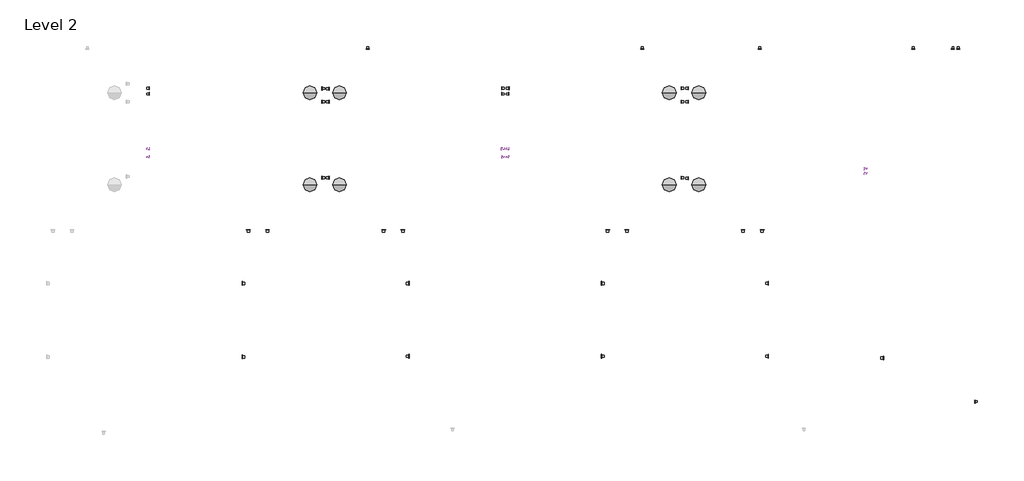
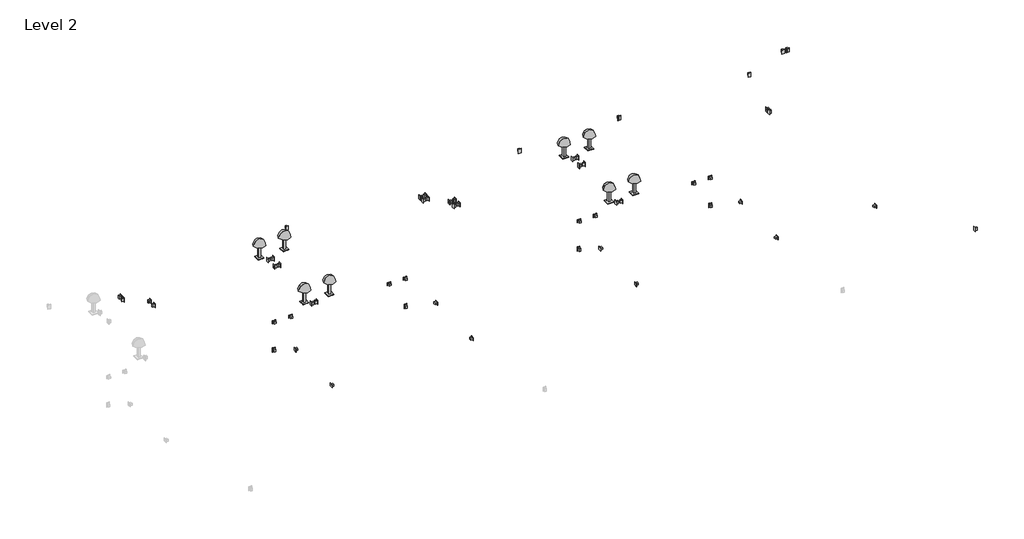
# One storey, part 2 of 2: 37 proxies, 17 switching devices, 8 light fixtures.
"""IFC4 building model written with IfcOpenShell, lengths in millimetres."""

import ifcopenshell
import ifcopenshell.guid

model = None  # the IFC model being written
_history = None  # IfcOwnerHistory: only IFC2X3 demands one
_inside = {}  # id of a spatial element -> (the spatial element, [elements in it])
_under = {}  # id of a project, library or spatial element -> (it, [spatial elements below it])
_declared = {}  # id of a project -> (the project, [libraries it declares])
_typed = {}  # id of a type object -> (the type object, [elements of that type])
_made_of = {}  # id of a material, layer set ... -> (it, [elements and type objects made of it])


def new_model(schema):
    """Start an empty IFC model of exactly this schema.

    Asked for "IFC4X3", IfcOpenShell would pick the latest addendum, in which some entities
    have other attributes; the version numbers below select the first issue.
    IFC2X3 requires an IfcOwnerHistory on every rooted entity: one is made here for all.
    """
    global model, _history
    if schema == "IFC4X3":
        model = ifcopenshell.file(schema_version=(4, 3, 0, 0))
    else:
        model = ifcopenshell.file(schema=schema)
    _inside.clear()
    _under.clear()
    _declared.clear()
    _typed.clear()
    _made_of.clear()
    _history = None
    if model.schema == "IFC2X3":
        org = make("IfcOrganization", Name="unknown")
        user = make(
            "IfcPersonAndOrganization",
            ThePerson=make("IfcPerson", FamilyName="unknown"),
            TheOrganization=org,
        )
        app = make(
            "IfcApplication",
            ApplicationDeveloper=org,
            Version="unknown",
            ApplicationFullName="unknown",
            ApplicationIdentifier="unknown",
        )
        _history = make(
            "IfcOwnerHistory",
            OwningUser=user,
            OwningApplication=app,
            ChangeAction="ADDED",
            CreationDate=0,
        )
    return model


def make(cls, **values):
    """One entity of the class cls with the attributes given. An attribute that is None is left unset."""
    return model.create_entity(
        cls, **{name: value for name, value in values.items() if value is not None}
    )


def rooted(cls, **values):
    """An entity with a GlobalId (a new one), such as an element, a storey or a relation."""
    return make(cls, GlobalId=ifcopenshell.guid.new(), OwnerHistory=_history, **values)


def si_unit(unit_type, name, prefix=None):
    """IfcSIUnit, for example si_unit("LENGTHUNIT", "METRE", prefix="MILLI")."""
    return make("IfcSIUnit", UnitType=unit_type, Prefix=prefix, Name=name)


def assignment(units):
    """IfcUnitAssignment: the units of a project."""
    return None if units is None else make("IfcUnitAssignment", Units=units)


def point(xyz):
    """IfcCartesianPoint."""
    return None if xyz is None else make("IfcCartesianPoint", Coordinates=xyz)


def direction(xyz):
    """IfcDirection."""
    return None if xyz is None else make("IfcDirection", DirectionRatios=xyz)


def frame(location, z_axis=None, x_axis=None):
    """IfcAxis2Placement3D, a coordinate frame: its origin and axes. An axis left out is left unset."""
    return make(
        "IfcAxis2Placement3D",
        Location=point(location),
        Axis=direction(z_axis),
        RefDirection=direction(x_axis),
    )


def frame_2d(location, x_axis=None):
    """IfcAxis2Placement2D, a coordinate frame in the plane: its origin and x axis."""
    return make(
        "IfcAxis2Placement2D", Location=point(location), RefDirection=direction(x_axis)
    )


def origin():
    """The frame at (0, 0, 0) with its axes left unset."""
    return frame((0.0, 0.0, 0.0))


def origin_with_axes():
    """The frame at (0, 0, 0) with the z axis (0, 0, 1) and the x axis (1, 0, 0) written out."""
    return frame((0.0, 0.0, 0.0), z_axis=(0.0, 0.0, 1.0), x_axis=(1.0, 0.0, 0.0))


def origin_2d():
    """The frame at (0, 0) in the plane with its x axis left unset."""
    return frame_2d((0.0, 0.0))


def place(relative_to, where):
    """IfcLocalPlacement: puts the frame where relative to a parent placement (None: the world)."""
    return make(
        "IfcLocalPlacement", PlacementRelTo=relative_to, RelativePlacement=where
    )


def context(
    kind, dimensions, precision=None, world=None, true_north=None, identifier=None
):
    """IfcGeometricRepresentationContext, for example the 3D "Model" context."""
    return make(
        "IfcGeometricRepresentationContext",
        ContextIdentifier=identifier,
        ContextType=kind,
        CoordinateSpaceDimension=dimensions,
        Precision=precision,
        WorldCoordinateSystem=world,
        TrueNorth=true_north,
    )


def project(units=None, contexts=None):
    """IfcProject with its units and contexts."""
    return rooted(
        "IfcProject",
        Name="project",
        RepresentationContexts=contexts,
        UnitsInContext=assignment(units),
    )


def spatial(cls, under=None, at=None, **own):
    """A site, building, storey or space (cls), placed at a placement, below another one or the project."""
    s = rooted(cls, ObjectPlacement=at, **own)
    if under is not None:
        _under.setdefault(under.id(), (under, []))[1].append(s)
    return s


def polyline(points):
    """IfcPolyline through the points."""
    return make("IfcPolyline", Points=[point(p) for p in points])


def circle_curve(where, radius):
    """IfcCircle in the frame where."""
    return make("IfcCircle", Position=where, Radius=radius)


def ellipse_curve(where, semi_axis1, semi_axis2):
    """IfcEllipse in the frame where."""
    return make(
        "IfcEllipse", Position=where, SemiAxis1=semi_axis1, SemiAxis2=semi_axis2
    )


def trimmed(basis, trim1, trim2, sense, master):
    """IfcTrimmedCurve: the piece of a basis curve between two trims."""
    return make(
        "IfcTrimmedCurve",
        BasisCurve=basis,
        Trim1=trim1,
        Trim2=trim2,
        SenseAgreement=sense,
        MasterRepresentation=master,
    )


def segment(curve, same_sense, transition):
    """IfcCompositeCurveSegment."""
    return make(
        "IfcCompositeCurveSegment",
        Transition=transition,
        SameSense=same_sense,
        ParentCurve=curve,
    )


def composite_curve(segments, self_intersect=None):
    """IfcCompositeCurve: segments joined end to end."""
    return make("IfcCompositeCurve", Segments=segments, SelfIntersect=self_intersect)


def outline(outer, holes=None, kind="AREA"):
    """IfcArbitraryClosedProfileDef: a profile drawn as a closed curve; with holes, ...WithVoids."""
    if holes is None:
        return make("IfcArbitraryClosedProfileDef", ProfileType=kind, OuterCurve=outer)
    return make(
        "IfcArbitraryProfileDefWithVoids",
        ProfileType=kind,
        OuterCurve=outer,
        InnerCurves=holes,
    )


def extrude(swept, where, along, depth):
    """IfcExtrudedAreaSolid: the profile swept, set in the frame where, extruded along a direction by depth."""
    return make(
        "IfcExtrudedAreaSolid",
        SweptArea=swept,
        Position=where,
        ExtrudedDirection=direction(along),
        Depth=depth,
    )


def shape(context_of_items, identifier, shape_type, items):
    """IfcShapeRepresentation: the items that make up one representation, for example the "Body"."""
    return make(
        "IfcShapeRepresentation",
        ContextOfItems=context_of_items,
        RepresentationIdentifier=identifier,
        RepresentationType=shape_type,
        Items=items,
    )


def source(mapping_origin, context_of_items, identifier, shape_type, items):
    """IfcRepresentationMap: a shape defined once, which mapped items show again and again."""
    return make(
        "IfcRepresentationMap",
        MappingOrigin=mapping_origin,
        MappedRepresentation=shape(context_of_items, identifier, shape_type, items),
    )


def transform(
    local_origin,
    x_axis=None,
    y_axis=None,
    z_axis=None,
    scale=None,
    scale2=None,
    scale3=None,
    uniform=True,
):
    """IfcCartesianTransformationOperator3D, or its non-uniform kind. x_axis, y_axis, z_axis: its Axis1, 2, 3."""
    if uniform:
        return make(
            "IfcCartesianTransformationOperator3D",
            Axis1=direction(x_axis),
            Axis2=direction(y_axis),
            LocalOrigin=point(local_origin),
            Scale=scale,
            Axis3=direction(z_axis),
        )
    return make(
        "IfcCartesianTransformationOperator3DnonUniform",
        Axis1=direction(x_axis),
        Axis2=direction(y_axis),
        LocalOrigin=point(local_origin),
        Scale=scale,
        Axis3=direction(z_axis),
        Scale2=scale2,
        Scale3=scale3,
    )


def mapped(mapping_source, mapping_target):
    """IfcMappedItem: shows the shape of a source again, moved by a transform."""
    return make(
        "IfcMappedItem", MappingSource=mapping_source, MappingTarget=mapping_target
    )


def made_of(thing, what):
    """Note that an element or type object is made of a material, layer set ...; save() writes the relation."""
    if what is not None:
        _made_of.setdefault(what.id(), (what, []))[1].append(thing)
    return thing


def element(
    cls,
    number,
    at=None,
    inside=None,
    cuts=None,
    type_object=None,
    material=None,
    context=None,
    identifier="Body",
    shape_type=None,
    held_by="IfcProductDefinitionShape",
    body=None,
    shapes=None,
    **own,
):
    """One element of the class cls, such as IfcWall. Its Tag is "e" and its number.

    at: its placement. inside: the storey or other place that contains it. cuts: it is an
    opening in that element (IfcRelVoidsElement). A single representation is given by context,
    identifier, shape_type and body (its items); several are given by shapes. held_by: the class
    of the entity that holds the representations. save() writes the other relations.
    """
    e = rooted(cls, Tag="e%d" % number, ObjectPlacement=at, **own)
    if body is not None:
        shapes = [shape(context, identifier, shape_type, body)]
    if shapes is not None:
        e.Representation = make(held_by, Representations=shapes)
    if inside is not None:
        _inside.setdefault(inside.id(), (inside, []))[1].append(e)
    if cuts is not None:
        rooted(
            "IfcRelVoidsElement", RelatingBuildingElement=cuts, RelatedOpeningElement=e
        )
    if type_object is not None:
        _typed.setdefault(type_object.id(), (type_object, []))[1].append(e)
    return made_of(e, material)


def aggregate(whole, parts):
    """IfcRelAggregates: a whole, such as a stair, and the parts it consists of."""
    return rooted("IfcRelAggregates", RelatingObject=whole, RelatedObjects=parts)


def save(model, path):
    """Write the relations noted so far, then the file.

    IfcRelAggregates (storeys below a building ...), IfcRelContainedInSpatialStructure (elements
    in a storey), IfcRelDefinesByType, IfcRelAssociatesMaterial and IfcRelDeclares: one each for
    every whole, place, type object, material and project.
    """
    for whole, parts in _under.values():
        aggregate(whole, parts)
    for where, things in _inside.values():
        rooted(
            "IfcRelContainedInSpatialStructure",
            RelatedElements=things,
            RelatingStructure=where,
        )
    for kind, things in _typed.values():
        rooted("IfcRelDefinesByType", RelatedObjects=things, RelatingType=kind)
    for what, things in _made_of.values():
        rooted("IfcRelAssociatesMaterial", RelatedObjects=things, RelatingMaterial=what)
    for by, libraries in _declared.values():
        rooted("IfcRelDeclares", RelatingContext=by, RelatedDefinitions=libraries)
    model.write(path)


def plane_surface(at):
    """IfcPlane: the flat surface through the origin of the frame at, square to its z axis."""
    return make("IfcPlane", Position=at)


def revolved_surface(curve, axis_point, axis_direction):
    """IfcSurfaceOfRevolution: the curve turned about the line through axis_point along axis_direction."""
    return make(
        "IfcSurfaceOfRevolution",
        SweptCurve=make("IfcArbitraryOpenProfileDef", ProfileType="CURVE", Curve=curve),
        AxisPosition=make("IfcAxis1Placement", Location=point(axis_point), Axis=direction(axis_direction)),
    )


def advanced_brep(points, edges, surfaces, faces):
    """IfcAdvancedBrep: a solid bounded by faces that lie on surfaces and meet in shared edges.

    An edge is (start, end): straight between two places in points (the first is 0);
    or (start, end, curve); or (start, end, curve, False) where it runs against its curve.
    A face is (place in surfaces, loops), or (place, loops, False) where it looks against
    its surface's normal. A loop lists edges by number (the first is 1), with a minus sign
    where the edge is run from its end to its start. The first loop is the outer one.
    """
    corners = [point(p) for p in points]
    vertices = [make("IfcVertexPoint", VertexGeometry=c) for c in corners]
    made = []
    for start, end, *more in edges:
        made.append(
            make(
                "IfcEdgeCurve",
                EdgeStart=vertices[start],
                EdgeEnd=vertices[end],
                EdgeGeometry=more[0] if more else make("IfcPolyline", Points=[corners[start], corners[end]]),
                SameSense=more[1] if len(more) > 1 else True,
            )
        )
    hull = []
    for where, loops, *sense in faces:
        bounds = []
        for j, loop in enumerate(loops):
            ring = [make("IfcOrientedEdge", EdgeElement=made[abs(k) - 1], Orientation=k > 0) for k in loop]
            bounds.append(
                make(
                    "IfcFaceOuterBound" if j == 0 else "IfcFaceBound",
                    Bound=make("IfcEdgeLoop", EdgeList=ring),
                    Orientation=True,
                )
            )
        hull.append(make("IfcAdvancedFace", Bounds=bounds, FaceSurface=surfaces[where], SameSense=sense[0] if sense else True))
    return make("IfcAdvancedBrep", Outer=make("IfcClosedShell", CfsFaces=hull))


def m_duplex_receptacle_top_switched_standard_10251bba(model_context):
    return source(origin(), model_context, "Body", "SweptSolid", [
        extrude(outline(polyline([(19.05, 38.1), (19.05, -38.1), (-19.05, -38.1), (-19.05, 38.1), (19.05, 38.1)])), frame((0.0, 0.0, -53.975), z_axis=(0.0, 0.0, 1.0), x_axis=(1.0, 0.0, 0.0)), (0.0, 0.0, 1.0), 53.975),
        extrude(outline(polyline([(34.925, 57.15), (34.925, -57.15), (-34.925, -57.15), (-34.925, 57.15), (34.925, 57.15)])), origin_with_axes(), (0.0, 0.0, 1.0), 4.7625),
    ])


def standard_8138c307(model_context):
    return source(origin(), model_context, "Body", "SweptSolid", [
        extrude(outline(polyline([(34.925, 57.15), (34.925, -57.15), (-34.925, -57.15), (-34.925, 57.15), (34.925, 57.15)]), holes=[composite_curve([segment(trimmed(circle_curve(frame_2d((0.6039572, -2.5749254)), 6.9441889), [point((-6.3402317, -2.5749254))], [point((7.5481461, -2.5749254))], True, "CARTESIAN"), True, "CONTINUOUS"), segment(trimmed(circle_curve(frame_2d((0.6039572, -2.5749254)), 6.9441889), [point((7.5481461, -2.5749254))], [point((-6.3402317, -2.5749254))], True, "CARTESIAN"), True, "CONTINUOUS")], self_intersect=False)]), origin_with_axes(), (0.0, 0.0, 1.0), 4.7625),
        extrude(outline(polyline([(19.05, 38.1), (19.05, -38.1), (-19.05, -38.1), (-19.05, 38.1), (19.05, 38.1)]), holes=[composite_curve([segment(trimmed(circle_curve(frame_2d((0.0, -0.79375)), 7.0675853), [point((-7.0675853, -0.79375))], [point((7.0675853, -0.79375))], True, "CARTESIAN"), True, "CONTINUOUS"), segment(trimmed(circle_curve(frame_2d((0.0, -0.79375)), 7.0675853), [point((7.0675853, -0.79375))], [point((-7.0675853, -0.79375))], True, "CARTESIAN"), True, "CONTINUOUS")], self_intersect=False)]), frame((0.0, 0.0, -53.975), z_axis=(0.0, 0.0, 1.0), x_axis=(1.0, 0.0, 0.0)), (0.0, 0.0, 1.0), 53.975),
    ])


def table_lamp_hemispheric_60w_230v_02721d88(model_context):
    return source(origin(), model_context, "Body", "SolidModel", [
        advanced_brep(
        [(0.0, 0.0, 524.5095504), (152.4, 0.0, 372.1095504), (-152.4, 0.0, 372.1095504), (-146.05, 0.0, 372.1095504), (146.05, 0.0, 372.1095504), (0.0, 0.0, 518.1595504)],
        [
            (0, 1, circle_curve(frame((0.0, 0.0, 372.1095504), z_axis=(0.0, 1.0, 0.0), x_axis=(1.0, 0.0, 0.0)), 152.4)),
            (1, 2, circle_curve(frame((0.0, 0.0, 372.1095504), z_axis=(0.0, 0.0, 1.0), x_axis=(1.0, 0.0, 0.0)), 152.4)),
            (2, 0, circle_curve(frame((0.0, 0.0, 372.1095504), z_axis=(0.0, 1.0, 0.0), x_axis=(-1.0, 0.0, 0.0)), 152.4)),
            (2, 1, circle_curve(frame((0.0, 0.0, 372.1095504), z_axis=(0.0, 0.0, 1.0), x_axis=(1.0, 0.0, 0.0)), 152.4)),
            (3, 4, circle_curve(frame((0.0, 0.0, 372.1095504), z_axis=(0.0, 0.0, -1.0), x_axis=(1.0, 0.0, 0.0)), 146.05)),
            (4, 5, circle_curve(frame((0.0, 0.0, 372.1095504), z_axis=(0.0, -1.0, 0.0), x_axis=(1.0, 0.0, 0.0)), 146.05)),
            (5, 3, circle_curve(frame((0.0, 0.0, 372.1095504), z_axis=(0.0, -1.0, 0.0), x_axis=(-1.0, 0.0, 0.0)), 146.05)),
            (4, 3, circle_curve(frame((0.0, 0.0, 372.1095504), z_axis=(0.0, 0.0, -1.0), x_axis=(1.0, 0.0, 0.0)), 146.05)),
            (1, 4),
            (3, 2),
        ],
        [
            revolved_surface(trimmed(ellipse_curve(frame((0.0, 0.0, 372.1095504), z_axis=(0.0, -1.0, 0.0), x_axis=(1.0, 0.0, 0.0)), 152.4, 152.4), [point((152.4, 0.0, 372.1095504))], [point((0.0, 0.0, 524.5095504))], True, "CARTESIAN"), (0.0, 0.0, 552.6321699), (0.0, 0.0, 1.0)),
            revolved_surface(trimmed(ellipse_curve(frame((0.0, 0.0, 372.1095504), z_axis=(0.0, 1.0, 0.0), x_axis=(1.0, 0.0, 0.0)), 146.05, 146.05), [point((0.0, 0.0, 518.1595504))], [point((146.05, 0.0, 372.1095504))], True, "CARTESIAN"), (0.0, 0.0, 552.6321699), (0.0, 0.0, 1.0)),
            plane_surface(frame((0.0, 0.0, 372.1095504), z_axis=(0.0, 0.0, -1.0), x_axis=(1.0, 0.0, 0.0))),
        ],
        [
            (0, [[1, 2, 3]]),
            (0, [[-3, 4, -1]]),
            (1, [[5, 6, 7]]),
            (1, [[8, -7, -6]]),
            (2, [[-2, 9, -5, 10]]),
            (2, [[-4, -10, -8, -9]]),
        ],
    ),
        extrude(outline(composite_curve([segment(trimmed(circle_curve(origin_2d(), 6.35), [point((-6.35, 0.0))], [point((6.35, 0.0))], False, "CARTESIAN"), True, "CONTINUOUS"), segment(trimmed(circle_curve(origin_2d(), 6.35), [point((6.35, 0.0))], [point((-6.35, 0.0))], False, "CARTESIAN"), True, "CONTINUOUS")], self_intersect=False)), frame((0.0, 0.0, 330.2), z_axis=(0.0, 0.0, 1.0), x_axis=(1.0, 0.0, 0.0)), (0.0, 0.0, 1.0), 63.5),
        extrude(outline(polyline([(25.4, -25.4), (-25.4, -25.4), (-25.4, 25.4), (25.4, 25.4), (25.4, -25.4)])), frame((0.0, 0.0, 25.4), z_axis=(0.0, 0.0, 1.0), x_axis=(1.0, 0.0, 0.0)), (0.0, 0.0, 1.0), 304.8),
        advanced_brep(
        [(-66.7336963, -50.8, 12.7), (-34.9836963, -50.8, 12.7), (-47.6836963, -50.8, 0.0), (-54.0336963, -50.8, 0.0), (-54.0336963, -50.8, 12.7), (-47.6836963, -50.8, 12.7)],
        [
            (0, 1, circle_curve(frame((-50.8586963, -50.8, 12.7), z_axis=(0.0, 0.0, -1.0), x_axis=(1.0, 0.0, 0.0)), 15.875)),
            (1, 2, circle_curve(frame((-47.6836963, -50.8, 12.7), z_axis=(0.0, 1.0, 0.0), x_axis=(1.0, 0.0, 0.0)), 12.7)),
            (2, 3, circle_curve(frame((-50.8586963, -50.8, 0.0), z_axis=(0.0, 0.0, 1.0), x_axis=(1.0, 0.0, 0.0)), 3.175)),
            (3, 0, circle_curve(frame((-54.0336963, -50.8, 12.7), z_axis=(0.0, 1.0, 0.0), x_axis=(-1.0, 0.0, 0.0)), 12.7)),
            (1, 0, circle_curve(frame((-50.8586963, -50.8, 12.7), z_axis=(0.0, 0.0, -1.0), x_axis=(1.0, 0.0, 0.0)), 15.875)),
            (3, 2, circle_curve(frame((-50.8586963, -50.8, 0.0), z_axis=(0.0, 0.0, 1.0), x_axis=(1.0, 0.0, 0.0)), 3.175)),
            (4, 5, circle_curve(frame((-50.8586963, -50.8, 12.7), z_axis=(0.0, 0.0, -1.0), x_axis=(1.0, 0.0, 0.0)), 3.175)),
            (5, 1),
            (0, 4),
            (5, 4, circle_curve(frame((-50.8586963, -50.8, 12.7), z_axis=(0.0, 0.0, -1.0), x_axis=(1.0, 0.0, 0.0)), 3.175)),
            (2, 5),
            (4, 3),
        ],
        [
            revolved_surface(trimmed(ellipse_curve(frame((-47.6836963, -50.8, 12.7), z_axis=(0.0, -1.0, 0.0), x_axis=(1.0, 0.0, 0.0)), 12.7, 12.7), [point((-47.6836963, -50.8, 0.0))], [point((-34.9836963, -50.8, 12.7))], True, "CARTESIAN"), (-50.8586963, -50.8, 36.0623287), (0.0, 0.0, 1.0)),
            plane_surface(frame((-50.8586963, -50.8, 12.7), z_axis=(0.0, 0.0, 1.0), x_axis=(1.0, 0.0, 0.0))),
            revolved_surface(polyline([(-47.6836963, -50.8, 12.7), (-47.6836963, -50.8, 0.0)]), (-50.8586963, -50.8, 36.0623287), (0.0, 0.0, 1.0)),
        ],
        [
            (0, [[1, 2, 3, 4]]),
            (0, [[5, -4, 6, -2]]),
            (1, [[7, 8, -1, 9]]),
            (1, [[10, -9, -5, -8]]),
            (2, [[-3, 11, -7, 12]]),
            (2, [[-6, -12, -10, -11]]),
        ],
    ),
        advanced_brep(
        [(-66.7581301, 50.8, 12.7), (-35.0081301, 50.8, 12.7), (-47.7081301, 50.8, 0.0), (-54.0581301, 50.8, 0.0), (-54.0581301, 50.8, 12.7), (-47.7081301, 50.8, 12.7)],
        [
            (0, 1, circle_curve(frame((-50.8831301, 50.8, 12.7), z_axis=(0.0, 0.0, -1.0), x_axis=(1.0, 0.0, 0.0)), 15.875)),
            (1, 2, circle_curve(frame((-47.7081301, 50.8, 12.7), z_axis=(0.0, 1.0, 0.0), x_axis=(1.0, 0.0, 0.0)), 12.7)),
            (2, 3, circle_curve(frame((-50.8831301, 50.8, 0.0), z_axis=(0.0, 0.0, 1.0), x_axis=(1.0, 0.0, 0.0)), 3.175)),
            (3, 0, circle_curve(frame((-54.0581301, 50.8, 12.7), z_axis=(0.0, 1.0, 0.0), x_axis=(-1.0, 0.0, 0.0)), 12.7)),
            (1, 0, circle_curve(frame((-50.8831301, 50.8, 12.7), z_axis=(0.0, 0.0, -1.0), x_axis=(1.0, 0.0, 0.0)), 15.875)),
            (3, 2, circle_curve(frame((-50.8831301, 50.8, 0.0), z_axis=(0.0, 0.0, 1.0), x_axis=(1.0, 0.0, 0.0)), 3.175)),
            (4, 5, circle_curve(frame((-50.8831301, 50.8, 12.7), z_axis=(0.0, 0.0, -1.0), x_axis=(1.0, 0.0, 0.0)), 3.175)),
            (5, 1),
            (0, 4),
            (5, 4, circle_curve(frame((-50.8831301, 50.8, 12.7), z_axis=(0.0, 0.0, -1.0), x_axis=(1.0, 0.0, 0.0)), 3.175)),
            (2, 5),
            (4, 3),
        ],
        [
            revolved_surface(trimmed(ellipse_curve(frame((-47.7081301, 50.8, 12.7), z_axis=(0.0, -1.0, 0.0), x_axis=(1.0, 0.0, 0.0)), 12.7, 12.7), [point((-47.7081301, 50.8, 0.0))], [point((-35.0081301, 50.8, 12.7))], True, "CARTESIAN"), (-50.8831301, 50.8, 36.0623287), (0.0, 0.0, 1.0)),
            plane_surface(frame((-50.8831301, 50.8, 12.7), z_axis=(0.0, 0.0, 1.0), x_axis=(1.0, 0.0, 0.0))),
            revolved_surface(polyline([(-47.708130100000005, 50.8, 12.7), (-47.708130100000005, 50.8, 0.0)]), (-50.8831301, 50.8, 36.0623287), (0.0, 0.0, 1.0)),
        ],
        [
            (0, [[1, 2, 3, 4]]),
            (0, [[5, -4, 6, -2]]),
            (1, [[7, 8, -1, 9]]),
            (1, [[10, -9, -5, -8]]),
            (2, [[-3, 11, -7, 12]]),
            (2, [[-6, -12, -10, -11]]),
        ],
    ),
        advanced_brep(
        [(34.9494337, -50.8, 12.7), (66.6994337, -50.8, 12.7), (53.9994337, -50.8, 0.0), (47.6494337, -50.8, 0.0), (47.6494337, -50.8, 12.7), (53.9994337, -50.8, 12.7)],
        [
            (0, 1, circle_curve(frame((50.8244337, -50.8, 12.7), z_axis=(0.0, 0.0, -1.0), x_axis=(1.0, 0.0, 0.0)), 15.875)),
            (1, 2, circle_curve(frame((53.9994337, -50.8, 12.7), z_axis=(0.0, 1.0, 0.0), x_axis=(1.0, 0.0, 0.0)), 12.7)),
            (2, 3, circle_curve(frame((50.8244337, -50.8, 0.0), z_axis=(0.0, 0.0, 1.0), x_axis=(1.0, 0.0, 0.0)), 3.175)),
            (3, 0, circle_curve(frame((47.6494337, -50.8, 12.7), z_axis=(0.0, 1.0, 0.0), x_axis=(-1.0, 0.0, 0.0)), 12.7)),
            (1, 0, circle_curve(frame((50.8244337, -50.8, 12.7), z_axis=(0.0, 0.0, -1.0), x_axis=(1.0, 0.0, 0.0)), 15.875)),
            (3, 2, circle_curve(frame((50.8244337, -50.8, 0.0), z_axis=(0.0, 0.0, 1.0), x_axis=(1.0, 0.0, 0.0)), 3.175)),
            (4, 5, circle_curve(frame((50.8244337, -50.8, 12.7), z_axis=(0.0, 0.0, -1.0), x_axis=(1.0, 0.0, 0.0)), 3.175)),
            (5, 1),
            (0, 4),
            (5, 4, circle_curve(frame((50.8244337, -50.8, 12.7), z_axis=(0.0, 0.0, -1.0), x_axis=(1.0, 0.0, 0.0)), 3.175)),
            (2, 5),
            (4, 3),
        ],
        [
            revolved_surface(trimmed(ellipse_curve(frame((53.9994337, -50.8, 12.7), z_axis=(0.0, -1.0, 0.0), x_axis=(1.0, 0.0, 0.0)), 12.7, 12.7), [point((53.9994337, -50.8, 0.0))], [point((66.6994337, -50.8, 12.7))], True, "CARTESIAN"), (50.8244337, -50.8, 36.0623287), (0.0, 0.0, 1.0)),
            plane_surface(frame((50.8244337, -50.8, 12.7), z_axis=(0.0, 0.0, 1.0), x_axis=(1.0, 0.0, 0.0))),
            revolved_surface(polyline([(53.9994337, -50.8, 12.7), (53.9994337, -50.8, 0.0)]), (50.8244337, -50.8, 36.0623287), (0.0, 0.0, 1.0)),
        ],
        [
            (0, [[1, 2, 3, 4]]),
            (0, [[5, -4, 6, -2]]),
            (1, [[7, 8, -1, 9]]),
            (1, [[10, -9, -5, -8]]),
            (2, [[-3, 11, -7, 12]]),
            (2, [[-6, -12, -10, -11]]),
        ],
    ),
        advanced_brep(
        [(34.925, 50.8, 12.7), (66.675, 50.8, 12.7), (53.975, 50.8, 0.0), (47.625, 50.8, 0.0), (47.625, 50.8, 12.7), (53.975, 50.8, 12.7)],
        [
            (0, 1, circle_curve(frame((50.8, 50.8, 12.7), z_axis=(0.0, 0.0, -1.0), x_axis=(1.0, 0.0, 0.0)), 15.875)),
            (1, 2, circle_curve(frame((53.975, 50.8, 12.7), z_axis=(0.0, 1.0, 0.0), x_axis=(1.0, 0.0, 0.0)), 12.7)),
            (2, 3, circle_curve(frame((50.8, 50.8, 0.0), z_axis=(0.0, 0.0, 1.0), x_axis=(1.0, 0.0, 0.0)), 3.175)),
            (3, 0, circle_curve(frame((47.625, 50.8, 12.7), z_axis=(0.0, 1.0, 0.0), x_axis=(-1.0, 0.0, 0.0)), 12.7)),
            (1, 0, circle_curve(frame((50.8, 50.8, 12.7), z_axis=(0.0, 0.0, -1.0), x_axis=(1.0, 0.0, 0.0)), 15.875)),
            (3, 2, circle_curve(frame((50.8, 50.8, 0.0), z_axis=(0.0, 0.0, 1.0), x_axis=(1.0, 0.0, 0.0)), 3.175)),
            (4, 5, circle_curve(frame((50.8, 50.8, 12.7), z_axis=(0.0, 0.0, -1.0), x_axis=(1.0, 0.0, 0.0)), 3.175)),
            (5, 1),
            (0, 4),
            (5, 4, circle_curve(frame((50.8, 50.8, 12.7), z_axis=(0.0, 0.0, -1.0), x_axis=(1.0, 0.0, 0.0)), 3.175)),
            (2, 5),
            (4, 3),
        ],
        [
            revolved_surface(trimmed(ellipse_curve(frame((53.975, 50.8, 12.7), z_axis=(0.0, -1.0, 0.0), x_axis=(1.0, 0.0, 0.0)), 12.7, 12.7), [point((53.975, 50.8, 0.0))], [point((66.675, 50.8, 12.7))], True, "CARTESIAN"), (50.8, 50.8, 36.0623287), (0.0, 0.0, 1.0)),
            plane_surface(frame((50.8, 50.8, 12.7), z_axis=(0.0, 0.0, 1.0), x_axis=(1.0, 0.0, 0.0))),
            revolved_surface(polyline([(53.974999999999994, 50.8, 12.7), (53.974999999999994, 50.8, 0.0)]), (50.8, 50.8, 36.0623287), (0.0, 0.0, 1.0)),
        ],
        [
            (0, [[1, 2, 3, 4]]),
            (0, [[5, -4, 6, -2]]),
            (1, [[7, 8, -1, 9]]),
            (1, [[10, -9, -5, -8]]),
            (2, [[-3, 11, -7, 12]]),
            (2, [[-6, -12, -10, -11]]),
        ],
    ),
        extrude(outline(polyline([(76.2, 76.2), (76.2, -76.2), (-76.2, -76.2), (-76.2, 76.2), (76.2, 76.2)])), frame((0.0, 0.0, 12.7), z_axis=(0.0, 0.0, 1.0), x_axis=(1.0, 0.0, 0.0)), (0.0, 0.0, 1.0), 12.7),
    ])


def lighting_switches_four_way_four_way_switch_ab144c04(model_context):
    return source(origin(), model_context, "Body", "SweptSolid", [
        extrude(outline(polyline([(43.0, -86.0), (-43.0, -86.0), (-43.0, 0.0), (43.0, 0.0), (43.0, -86.0)])), origin_with_axes(), (0.0, 0.0, 1.0), 5.0),
        extrude(outline(polyline([(27.0, -67.0), (-27.0, -67.0), (-27.0, -19.0), (27.0, -19.0), (27.0, -67.0)])), frame((0.0, 0.0, -54.0), z_axis=(0.0, 0.0, 1.0), x_axis=(1.0, 0.0, 0.0)), (0.0, 0.0, 1.0), 54.0),
    ])


model = new_model("IFC4")

# Units and contexts
model_context = context("Model", 3, world=origin())
ifc_project = project(units=[si_unit("LENGTHUNIT", "METRE", prefix="MILLI")], contexts=[model_context])

# Site, building, storey
site = spatial("IfcSite", under=ifc_project)
building = spatial("IfcBuilding", under=site)
storey = spatial("IfcBuildingStorey", under=building, Name="Level 2", Elevation=103800.0)

# Proxies
placement = place(None, origin())
m_duplex_receptacle_top_switched_standard_shape = m_duplex_receptacle_top_switched_standard_10251bba(model_context)
element("IfcBuildingElementProxy", 1, Name="M_Duplex Receptacle - Top Switched : Standard", ObjectType="M_Duplex Receptacle - Top Switched : Standard", at=placement, inside=storey, context=model_context, shape_type="MappedRepresentation", body=[
    mapped(m_duplex_receptacle_top_switched_standard_shape, transform((28197.0017353, 13930.039, 104190.0), x_axis=(0.0, -1.0, 0.0), y_axis=(0.0, 0.0, 1.0), z_axis=(-1.0, 0.0, 0.0))),
])
element("IfcBuildingElementProxy", 2, Name="M_Duplex Receptacle - Top Switched : Standard", ObjectType="M_Duplex Receptacle - Top Switched : Standard", at=placement, inside=storey, context=model_context, shape_type="MappedRepresentation", body=[
    mapped(m_duplex_receptacle_top_switched_standard_shape, transform((28347.0017353, 13930.039, 104190.0), x_axis=(0.0, 1.0, 0.0), y_axis=(0.0, 0.0, 1.0), z_axis=(1.0, 0.0, 0.0))),
])
element("IfcBuildingElementProxy", 3, Name="M_Duplex Receptacle - Top Switched : Standard", ObjectType="M_Duplex Receptacle - Top Switched : Standard", at=placement, inside=storey, context=model_context, shape_type="MappedRepresentation", body=[
    mapped(m_duplex_receptacle_top_switched_standard_shape, transform((28347.0017353, 12235.1140001, 104190.0), x_axis=(0.0, 1.0, 0.0), y_axis=(0.0, 0.0, 1.0), z_axis=(1.0, 0.0, 0.0))),
])
element("IfcBuildingElementProxy", 4, Name="M_Duplex Receptacle - Top Switched : Standard", ObjectType="M_Duplex Receptacle - Top Switched : Standard", at=placement, inside=storey, context=model_context, shape_type="MappedRepresentation", body=[
    mapped(m_duplex_receptacle_top_switched_standard_shape, transform((20389.0307208, 13930.039, 104190.0), x_axis=(0.0, 1.0, 0.0), y_axis=(0.0, 0.0, 1.0), z_axis=(1.0, 0.0, 0.0))),
])
element("IfcBuildingElementProxy", 5, Name="M_Duplex Receptacle - Top Switched : Standard", ObjectType="M_Duplex Receptacle - Top Switched : Standard", at=placement, inside=storey, context=model_context, shape_type="MappedRepresentation", body=[
    mapped(m_duplex_receptacle_top_switched_standard_shape, transform((20389.0307208, 12250.0390001, 104190.0), x_axis=(0.0, 1.0, 0.0), y_axis=(0.0, 0.0, 1.0), z_axis=(1.0, 0.0, 0.0))),
])
element("IfcBuildingElementProxy", 6, Name="M_Duplex Receptacle - Top Switched : Standard", ObjectType="M_Duplex Receptacle - Top Switched : Standard", at=placement, inside=storey, context=model_context, shape_type="MappedRepresentation", body=[
    mapped(m_duplex_receptacle_top_switched_standard_shape, transform((20239.0307208, 13930.039, 104190.0), x_axis=(0.0, -1.0, 0.0), y_axis=(0.0, 0.0, 1.0), z_axis=(-1.0, 0.0, 0.0))),
])
element("IfcBuildingElementProxy", 7, Name="M_Duplex Receptacle - Top Switched : Standard", ObjectType="M_Duplex Receptacle - Top Switched : Standard", at=placement, inside=storey, context=model_context, shape_type="MappedRepresentation", body=[
    mapped(m_duplex_receptacle_top_switched_standard_shape, transform((20239.0307208, 12250.0390001, 104190.0), x_axis=(0.0, -1.0, 0.0), y_axis=(0.0, 0.0, 1.0), z_axis=(-1.0, 0.0, 0.0))),
])
element("IfcBuildingElementProxy", 8, Name="M_Duplex Receptacle - Top Switched : Standard", ObjectType="M_Duplex Receptacle - Top Switched : Standard", at=placement, inside=storey, context=model_context, shape_type="MappedRepresentation", body=[
    mapped(m_duplex_receptacle_top_switched_standard_shape, transform((24369.0753139, 14105.0005078, 104520.0), x_axis=(0.0, 1.0, 0.0), y_axis=(0.0, 0.0, 1.0), z_axis=(1.0, 0.0, 0.0))),
])
element("IfcBuildingElementProxy", 9, Name="M_Duplex Receptacle - Top Switched : Standard", ObjectType="M_Duplex Receptacle - Top Switched : Standard", at=placement, inside=storey, context=model_context, shape_type="MappedRepresentation", body=[
    mapped(m_duplex_receptacle_top_switched_standard_shape, transform((28197.0017353, 12250.0390001, 104190.0), x_axis=(0.0, -1.0, 0.0), y_axis=(0.0, 0.0, 1.0), z_axis=(-1.0, 0.0, 0.0))),
])
element("IfcBuildingElementProxy", 10, Name="M_Duplex Receptacle - Top Switched : Standard", ObjectType="M_Duplex Receptacle - Top Switched : Standard", at=placement, inside=storey, context=model_context, shape_type="MappedRepresentation", body=[
    mapped(m_duplex_receptacle_top_switched_standard_shape, transform((34330.0000096, 15100.039, 104520.0), x_axis=(1.0, 0.0, 0.0), y_axis=(0.0, 0.0, 1.0), z_axis=(0.0, -1.0, 0.0))),
])
element("IfcBuildingElementProxy", 11, Name="M_Receptacle - 220V : Standard", ObjectType="M_Receptacle - 220V : Standard", at=placement, inside=storey, context=model_context, shape_type="MappedRepresentation", body=[
    mapped(m_duplex_receptacle_top_switched_standard_shape, transform((29930.005, 15100.039, 104190.0), x_axis=(1.0, 0.0, 0.0), y_axis=(0.0, 0.0, 1.0), z_axis=(0.0, -1.0, 0.0))),
])
element("IfcBuildingElementProxy", 12, Name="M_Receptacle - 220V : Standard", ObjectType="M_Receptacle - 220V : Standard", at=placement, inside=storey, context=model_context, shape_type="MappedRepresentation", body=[
    mapped(m_duplex_receptacle_top_switched_standard_shape, transform((33330.005, 15100.039, 104190.0), x_axis=(1.0, 0.0, 0.0), y_axis=(0.0, 0.0, 1.0), z_axis=(0.0, -1.0, 0.0))),
])
element("IfcBuildingElementProxy", 13, Name="M_Receptacle - 220V : Standard", ObjectType="M_Receptacle - 220V : Standard", at=placement, inside=storey, context=model_context, shape_type="MappedRepresentation", body=[
    mapped(m_duplex_receptacle_top_switched_standard_shape, transform((32250.005, 12350.0390001, 105212.0), x_axis=(0.0, -1.0, 0.0), y_axis=(0.0, 0.0, 1.0), z_axis=(-1.0, 0.0, 0.0))),
])
element("IfcBuildingElementProxy", 14, Name="M_Receptacle - 220V : Standard", ObjectType="M_Receptacle - 220V : Standard", at=placement, inside=storey, context=model_context, shape_type="MappedRepresentation", body=[
    mapped(m_duplex_receptacle_top_switched_standard_shape, transform((29992.6879533, 11096.4090428, 104190.0), x_axis=(-1.0, 0.0, 0.0), y_axis=(0.0, 0.0, 1.0), z_axis=(0.0, 1.0, 0.0))),
])
element("IfcBuildingElementProxy", 15, Name="M_Receptacle - 220V : Standard", ObjectType="M_Receptacle - 220V : Standard", at=placement, inside=storey, context=model_context, shape_type="MappedRepresentation", body=[
    mapped(m_duplex_receptacle_top_switched_standard_shape, transform((26556.2764984, 11096.4090428, 104190.0), x_axis=(-1.0, 0.0, 0.0), y_axis=(0.0, 0.0, 1.0), z_axis=(0.0, 1.0, 0.0))),
])
element("IfcBuildingElementProxy", 16, Name="M_Receptacle - 220V : Standard", ObjectType="M_Receptacle - 220V : Standard", at=placement, inside=storey, context=model_context, shape_type="MappedRepresentation", body=[
    mapped(m_duplex_receptacle_top_switched_standard_shape, transform((27330.005, 15100.039, 104190.0), x_axis=(1.0, 0.0, 0.0), y_axis=(0.0, 0.0, 1.0), z_axis=(0.0, -1.0, 0.0))),
])
element("IfcBuildingElementProxy", 17, Name="M_Receptacle - 220V : Standard", ObjectType="M_Receptacle - 220V : Standard", at=placement, inside=storey, context=model_context, shape_type="MappedRepresentation", body=[
    mapped(m_duplex_receptacle_top_switched_standard_shape, transform((24369.0753139, 12710.0390001, 105212.0), x_axis=(0.0, 1.0, 0.0), y_axis=(0.0, 0.0, 1.0), z_axis=(1.0, 0.0, 0.0))),
])
element("IfcBuildingElementProxy", 18, Name="M_Receptacle - 220V : Standard", ObjectType="M_Receptacle - 220V : Standard", at=placement, inside=storey, context=model_context, shape_type="MappedRepresentation", body=[
    mapped(m_duplex_receptacle_top_switched_standard_shape, transform((24219.0753139, 14105.0005078, 104520.0), x_axis=(0.0, -1.0, 0.0), y_axis=(0.0, 0.0, 1.0), z_axis=(-1.0, 0.0, 0.0))),
])
element("IfcBuildingElementProxy", 19, Name="M_Receptacle - 220V : Standard", ObjectType="M_Receptacle - 220V : Standard", at=placement, inside=storey, context=model_context, shape_type="MappedRepresentation", body=[
    mapped(m_duplex_receptacle_top_switched_standard_shape, transform((24219.0753139, 12710.0390001, 105212.0), x_axis=(0.0, -1.0, 0.0), y_axis=(0.0, 0.0, 1.0), z_axis=(-1.0, 0.0, 0.0))),
])
element("IfcBuildingElementProxy", 20, Name="M_Receptacle - 220V : Standard", ObjectType="M_Receptacle - 220V : Standard", at=placement, inside=storey, context=model_context, shape_type="MappedRepresentation", body=[
    mapped(m_duplex_receptacle_top_switched_standard_shape, transform((22034.7169388, 11096.4090428, 104190.0), x_axis=(-1.0, 0.0, 0.0), y_axis=(0.0, 0.0, 1.0), z_axis=(0.0, 1.0, 0.0))),
])
element("IfcBuildingElementProxy", 21, Name="M_Receptacle - 220V : Standard", ObjectType="M_Receptacle - 220V : Standard", at=placement, inside=storey, context=model_context, shape_type="MappedRepresentation", body=[
    mapped(m_duplex_receptacle_top_switched_standard_shape, transform((21251.8163786, 15100.039, 104190.0), x_axis=(1.0, 0.0, 0.0), y_axis=(0.0, 0.0, 1.0), z_axis=(0.0, -1.0, 0.0))),
])
element("IfcBuildingElementProxy", 22, Name="M_Receptacle - 220V : Standard", ObjectType="M_Receptacle - 220V : Standard", at=placement, inside=storey, context=model_context, shape_type="MappedRepresentation", body=[
    mapped(m_duplex_receptacle_top_switched_standard_shape, transform((16410.005, 14105.0005078, 104520.0), x_axis=(0.0, 1.0, 0.0), y_axis=(0.0, 0.0, 1.0), z_axis=(1.0, 0.0, 0.0))),
])
element("IfcBuildingElementProxy", 23, Name="M_Receptacle - 220V : Standard", ObjectType="M_Receptacle - 220V : Standard", at=placement, inside=storey, context=model_context, shape_type="MappedRepresentation", body=[
    mapped(m_duplex_receptacle_top_switched_standard_shape, transform((16410.005, 12710.0390001, 105212.0), x_axis=(0.0, 1.0, 0.0), y_axis=(0.0, 0.0, 1.0), z_axis=(1.0, 0.0, 0.0))),
])
element("IfcBuildingElementProxy", 24, Name="M_Receptacle - 220V : Standard", ObjectType="M_Receptacle - 220V : Standard", at=placement, inside=storey, context=model_context, shape_type="MappedRepresentation", body=[
    mapped(m_duplex_receptacle_top_switched_standard_shape, transform((18598.3054839, 11096.4090428, 104190.0), x_axis=(-1.0, 0.0, 0.0), y_axis=(0.0, 0.0, 1.0), z_axis=(0.0, 1.0, 0.0))),
])
element("IfcBuildingElementProxy", 25, Name="M_Receptacle - 220V : Standard", ObjectType="M_Receptacle - 220V : Standard", at=placement, inside=storey, context=model_context, shape_type="MappedRepresentation", body=[
    mapped(m_duplex_receptacle_top_switched_standard_shape, transform((34700.005, 7290.0390001, 104190.0), x_axis=(0.0, -1.0, 0.0), y_axis=(0.0, 0.0, 1.0), z_axis=(-1.0, 0.0, 0.0))),
])
element("IfcBuildingElementProxy", 26, Name="M_Receptacle - DATA socket : Standard", ObjectType="M_Receptacle - DATA socket : Standard", at=placement, inside=storey, context=model_context, shape_type="MappedRepresentation", body=[
    mapped(m_duplex_receptacle_top_switched_standard_shape, transform((16410.005, 14230.039, 104520.0), x_axis=(0.0, 1.0, 0.0), y_axis=(0.0, 0.0, 1.0), z_axis=(1.0, 0.0, 0.0))),
])
element("IfcBuildingElementProxy", 27, Name="M_Receptacle - DATA socket : Standard", ObjectType="M_Receptacle - DATA socket : Standard", at=placement, inside=storey, context=model_context, shape_type="MappedRepresentation", body=[
    mapped(m_duplex_receptacle_top_switched_standard_shape, transform((20239.0307208, 14225.6506439, 104190.0), x_axis=(0.0, -1.0, 0.0), y_axis=(0.0, 0.0, 1.0), z_axis=(-1.0, 0.0, 0.0))),
])
element("IfcBuildingElementProxy", 28, Name="M_Receptacle - DATA socket : Standard", ObjectType="M_Receptacle - DATA socket : Standard", at=placement, inside=storey, context=model_context, shape_type="MappedRepresentation", body=[
    mapped(m_duplex_receptacle_top_switched_standard_shape, transform((20389.0307208, 14219.1753837, 104190.0), x_axis=(0.0, 1.0, 0.0), y_axis=(0.0, 0.0, 1.0), z_axis=(1.0, 0.0, 0.0))),
])
element("IfcBuildingElementProxy", 29, Name="M_Receptacle - DATA socket : Standard", ObjectType="M_Receptacle - DATA socket : Standard", at=placement, inside=storey, context=model_context, shape_type="MappedRepresentation", body=[
    mapped(m_duplex_receptacle_top_switched_standard_shape, transform((24219.0753139, 14230.039, 104520.0), x_axis=(0.0, -1.0, 0.0), y_axis=(0.0, 0.0, 1.0), z_axis=(-1.0, 0.0, 0.0))),
])
element("IfcBuildingElementProxy", 30, Name="M_Receptacle - DATA socket : Standard", ObjectType="M_Receptacle - DATA socket : Standard", at=placement, inside=storey, context=model_context, shape_type="MappedRepresentation", body=[
    mapped(m_duplex_receptacle_top_switched_standard_shape, transform((28197.0017353, 14230.039, 104190.0), x_axis=(0.0, -1.0, 0.0), y_axis=(0.0, 0.0, 1.0), z_axis=(-1.0, 0.0, 0.0))),
])
element("IfcBuildingElementProxy", 31, Name="M_Receptacle - DATA socket : Standard", ObjectType="M_Receptacle - DATA socket : Standard", at=placement, inside=storey, context=model_context, shape_type="MappedRepresentation", body=[
    mapped(m_duplex_receptacle_top_switched_standard_shape, transform((34210.0000096, 15100.039, 104520.0), x_axis=(1.0, 0.0, 0.0), y_axis=(0.0, 0.0, 1.0), z_axis=(0.0, -1.0, 0.0))),
])
element("IfcBuildingElementProxy", 32, Name="M_Receptacle - DATA socket : Standard", ObjectType="M_Receptacle - DATA socket : Standard", at=placement, inside=storey, context=model_context, shape_type="MappedRepresentation", body=[
    mapped(m_duplex_receptacle_top_switched_standard_shape, transform((24373.8378139, 14230.039, 104520.0), x_axis=(0.0, 1.0, 0.0), y_axis=(0.0, 0.0, 1.0), z_axis=(1.0, 0.0, 0.0))),
])
element("IfcBuildingElementProxy", 33, Name="M_Receptacle - DATA socket : Standard", ObjectType="M_Receptacle - DATA socket : Standard", at=placement, inside=storey, context=model_context, shape_type="MappedRepresentation", body=[
    mapped(m_duplex_receptacle_top_switched_standard_shape, transform((28347.0017353, 14230.039, 104190.0), x_axis=(0.0, 1.0, 0.0), y_axis=(0.0, 0.0, 1.0), z_axis=(1.0, 0.0, 0.0))),
])
standard_shape = standard_8138c307(model_context)
element("IfcBuildingElementProxy", 34, Name="M_Receptacle -TV /Satellite Socket : Standard", ObjectType="M_Receptacle -TV /Satellite Socket : Standard", at=placement, inside=storey, context=model_context, shape_type="MappedRepresentation", body=[
    mapped(standard_shape, transform((24214.3128139, 12890.0390001, 105212.0), x_axis=(0.0, -1.0, 0.0), y_axis=(0.0, 0.0, 1.0), z_axis=(-1.0, 0.0, 0.0))),
])
element("IfcBuildingElementProxy", 35, Name="M_Receptacle -TV /Satellite Socket : Standard", ObjectType="M_Receptacle -TV /Satellite Socket : Standard", at=placement, inside=storey, context=model_context, shape_type="MappedRepresentation", body=[
    mapped(standard_shape, transform((24369.0753139, 12890.0390001, 105212.0), x_axis=(0.0, 1.0, 0.0), y_axis=(0.0, 0.0, 1.0), z_axis=(1.0, 0.0, 0.0))),
])
element("IfcBuildingElementProxy", 36, Name="M_Receptacle -TV /Satellite Socket : Standard", ObjectType="M_Receptacle -TV /Satellite Socket : Standard", at=placement, inside=storey, context=model_context, shape_type="MappedRepresentation", body=[
    mapped(standard_shape, transform((32250.005, 12450.0390001, 105212.0), x_axis=(0.0, -1.0, 0.0), y_axis=(0.0, 0.0, 1.0), z_axis=(-1.0, 0.0, 0.0))),
])
element("IfcBuildingElementProxy", 37, Name="M_Receptacle -TV /Satellite Socket : Standard", ObjectType="M_Receptacle -TV /Satellite Socket : Standard", at=placement, inside=storey, context=model_context, shape_type="MappedRepresentation", body=[
    mapped(standard_shape, transform((16410.005, 12890.0390001, 105212.0), x_axis=(0.0, 1.0, 0.0), y_axis=(0.0, 0.0, 1.0), z_axis=(1.0, 0.0, 0.0))),
])

# Light fixtures
table_lamp_hemispheric_60w_230v_shape = table_lamp_hemispheric_60w_230v_02721d88(model_context)
element("IfcLightFixture", 38, ObjectType="Table Lamp - Hemispheric : 60W - 230V", at=placement, inside=storey, context=model_context, shape_type="MappedRepresentation", body=[
    mapped(table_lamp_hemispheric_60w_230v_shape, transform((20623.0693481, 12093.9035022, 104400.0), x_axis=(1.0, 0.0, 0.0), y_axis=(0.0, 1.0, 0.0), z_axis=(0.0, 0.0, 1.0))),
])
element("IfcLightFixture", 39, ObjectType="Table Lamp - Hemispheric : 60W - 230V", at=placement, inside=storey, context=model_context, shape_type="MappedRepresentation", body=[
    mapped(table_lamp_hemispheric_60w_230v_shape, transform((20623.0693481, 14131.1951689, 104400.0), x_axis=(1.0, 0.0, 0.0), y_axis=(0.0, 1.0, 0.0), z_axis=(0.0, 0.0, 1.0))),
])
element("IfcLightFixture", 40, ObjectType="Table Lamp - Hemispheric : 60W - 230V", at=placement, inside=storey, context=model_context, shape_type="MappedRepresentation", body=[
    mapped(table_lamp_hemispheric_60w_230v_shape, transform((19968.8000616, 12093.9035022, 104400.0), x_axis=(1.0, 0.0, 0.0), y_axis=(0.0, 1.0, 0.0), z_axis=(0.0, 0.0, 1.0))),
])
element("IfcLightFixture", 41, ObjectType="Table Lamp - Hemispheric : 60W - 230V", at=placement, inside=storey, context=model_context, shape_type="MappedRepresentation", body=[
    mapped(table_lamp_hemispheric_60w_230v_shape, transform((19968.8000616, 14131.1951689, 104400.0), x_axis=(1.0, 0.0, 0.0), y_axis=(0.0, 1.0, 0.0), z_axis=(0.0, 0.0, 1.0))),
])
element("IfcLightFixture", 42, ObjectType="Table Lamp - Hemispheric : 60W - 230V", at=placement, inside=storey, context=model_context, shape_type="MappedRepresentation", body=[
    mapped(table_lamp_hemispheric_60w_230v_shape, transform((27926.7710761, 12093.9035022, 104400.0), x_axis=(1.0, 0.0, 0.0), y_axis=(0.0, 1.0, 0.0), z_axis=(0.0, 0.0, 1.0))),
])
element("IfcLightFixture", 43, ObjectType="Table Lamp - Hemispheric : 60W - 230V", at=placement, inside=storey, context=model_context, shape_type="MappedRepresentation", body=[
    mapped(table_lamp_hemispheric_60w_230v_shape, transform((27926.7710761, 14131.1951689, 104400.0), x_axis=(1.0, 0.0, 0.0), y_axis=(0.0, 1.0, 0.0), z_axis=(0.0, 0.0, 1.0))),
])
element("IfcLightFixture", 44, ObjectType="Table Lamp - Hemispheric : 60W - 230V", at=placement, inside=storey, context=model_context, shape_type="MappedRepresentation", body=[
    mapped(table_lamp_hemispheric_60w_230v_shape, transform((28581.0403626, 12093.9035022, 104400.0), x_axis=(1.0, 0.0, 0.0), y_axis=(0.0, 1.0, 0.0), z_axis=(0.0, 0.0, 1.0))),
])
element("IfcLightFixture", 45, ObjectType="Table Lamp - Hemispheric : 60W - 230V", at=placement, inside=storey, context=model_context, shape_type="MappedRepresentation", body=[
    mapped(table_lamp_hemispheric_60w_230v_shape, transform((28581.0403626, 14131.1951689, 104400.0), x_axis=(1.0, 0.0, 0.0), y_axis=(0.0, 1.0, 0.0), z_axis=(0.0, 0.0, 1.0))),
])

# Switching devices
lighting_switches_four_way_four_way_switch_shape = lighting_switches_four_way_four_way_switch_ab144c04(model_context)
element("IfcSwitchingDevice", 46, ObjectType="Lighting Switches One Way : One Way Switch", at=placement, inside=storey, context=model_context, shape_type="MappedRepresentation", body=[
    mapped(lighting_switches_four_way_four_way_switch_shape, transform((26429.3514984, 9910.5820743, 105000.0), x_axis=(0.0, -1.0, 0.0), y_axis=(0.0, 0.0, 1.0), z_axis=(-1.0, 0.0, 0.0))),
])
element("IfcSwitchingDevice", 47, ObjectType="Lighting Switches One Way : One Way Switch", at=placement, inside=storey, context=model_context, shape_type="MappedRepresentation", body=[
    mapped(lighting_switches_four_way_four_way_switch_shape, transform((30119.6129533, 9911.1238803, 105000.0), x_axis=(0.0, 1.0, 0.0), y_axis=(0.0, 0.0, 1.0), z_axis=(1.0, 0.0, 0.0))),
])
element("IfcSwitchingDevice", 48, ObjectType="Lighting Switches One Way : One Way Switch", at=placement, inside=storey, context=model_context, shape_type="MappedRepresentation", body=[
    mapped(lighting_switches_four_way_four_way_switch_shape, transform((22161.6419388, 9910.5820743, 105000.0), x_axis=(0.0, 1.0, 0.0), y_axis=(0.0, 0.0, 1.0), z_axis=(1.0, 0.0, 0.0))),
])
element("IfcSwitchingDevice", 49, ObjectType="Lighting Switches One Way : One Way Switch", at=placement, inside=storey, context=model_context, shape_type="MappedRepresentation", body=[
    mapped(lighting_switches_four_way_four_way_switch_shape, transform((18471.3804839, 9910.5820743, 105000.0), x_axis=(0.0, -1.0, 0.0), y_axis=(0.0, 0.0, 1.0), z_axis=(-1.0, 0.0, 0.0))),
])
element("IfcSwitchingDevice", 50, ObjectType="Lighting Switches One Way : One Way Switch", at=placement, inside=storey, context=model_context, shape_type="MappedRepresentation", body=[
    mapped(lighting_switches_four_way_four_way_switch_shape, transform((18606.3804839, 11096.4090428, 105000.0), x_axis=(-1.0, 0.0, 0.0), y_axis=(0.0, 0.0, 1.0), z_axis=(0.0, 1.0, 0.0))),
])
element("IfcSwitchingDevice", 51, ObjectType="Lighting Switches One Way : One Way Switch", at=placement, inside=storey, context=model_context, shape_type="MappedRepresentation", body=[
    mapped(lighting_switches_four_way_four_way_switch_shape, transform((19029.3804839, 11096.4090428, 105000.0), x_axis=(-1.0, 0.0, 0.0), y_axis=(0.0, 0.0, 1.0), z_axis=(0.0, 1.0, 0.0))),
])
element("IfcSwitchingDevice", 52, ObjectType="Lighting Switches One Way : One Way Switch", at=placement, inside=storey, context=model_context, shape_type="MappedRepresentation", body=[
    mapped(lighting_switches_four_way_four_way_switch_shape, transform((26987.3514984, 11096.4090428, 105000.0), x_axis=(-1.0, 0.0, 0.0), y_axis=(0.0, 0.0, 1.0), z_axis=(0.0, 1.0, 0.0))),
])
element("IfcSwitchingDevice", 53, ObjectType="Lighting Switches One Way : One Way Switch", at=placement, inside=storey, context=model_context, shape_type="MappedRepresentation", body=[
    mapped(lighting_switches_four_way_four_way_switch_shape, transform((29561.6129533, 11096.4090428, 105000.0), x_axis=(-1.0, 0.0, 0.0), y_axis=(0.0, 0.0, 1.0), z_axis=(0.0, 1.0, 0.0))),
])
element("IfcSwitchingDevice", 54, ObjectType="Lighting Switches One Way : One Way Switch", at=placement, inside=storey, context=model_context, shape_type="MappedRepresentation", body=[
    mapped(lighting_switches_four_way_four_way_switch_shape, transform((29984.6129533, 11096.4090428, 105000.0), x_axis=(-1.0, 0.0, 0.0), y_axis=(0.0, 0.0, 1.0), z_axis=(0.0, 1.0, 0.0))),
])
element("IfcSwitchingDevice", 55, ObjectType="Lighting Switches One Way : One Way Switch", at=placement, inside=storey, context=model_context, shape_type="MappedRepresentation", body=[
    mapped(lighting_switches_four_way_four_way_switch_shape, transform((18471.3804839, 8280.4056984, 105000.0), x_axis=(0.0, -1.0, 0.0), y_axis=(0.0, 0.0, 1.0), z_axis=(-1.0, 0.0, 0.0))),
])
element("IfcSwitchingDevice", 56, ObjectType="Lighting Switches One Way : One Way Switch", at=placement, inside=storey, context=model_context, shape_type="MappedRepresentation", body=[
    mapped(lighting_switches_four_way_four_way_switch_shape, transform((22161.6419388, 8294.4056984, 105000.0), x_axis=(0.0, 1.0, 0.0), y_axis=(0.0, 0.0, 1.0), z_axis=(1.0, 0.0, 0.0))),
])
element("IfcSwitchingDevice", 57, ObjectType="Lighting Switches One Way : One Way Switch", at=placement, inside=storey, context=model_context, shape_type="MappedRepresentation", body=[
    mapped(lighting_switches_four_way_four_way_switch_shape, transform((26429.3514984, 8294.4056984, 105000.0), x_axis=(0.0, -1.0, 0.0), y_axis=(0.0, 0.0, 1.0), z_axis=(-1.0, 0.0, 0.0))),
])
element("IfcSwitchingDevice", 58, ObjectType="Lighting Switches One Way : One Way Switch", at=placement, inside=storey, context=model_context, shape_type="MappedRepresentation", body=[
    mapped(lighting_switches_four_way_four_way_switch_shape, transform((30119.6129533, 8294.4056984, 105000.0), x_axis=(0.0, 1.0, 0.0), y_axis=(0.0, 0.0, 1.0), z_axis=(1.0, 0.0, 0.0))),
])
element("IfcSwitchingDevice", 59, ObjectType="Lighting Switches One Way : One Way Switch", at=placement, inside=storey, context=model_context, shape_type="MappedRepresentation", body=[
    mapped(lighting_switches_four_way_four_way_switch_shape, transform((21603.6419388, 11096.4090428, 105000.0), x_axis=(-1.0, 0.0, 0.0), y_axis=(0.0, 0.0, 1.0), z_axis=(0.0, 1.0, 0.0))),
])
element("IfcSwitchingDevice", 60, ObjectType="Lighting Switches One Way : One Way Switch", at=placement, inside=storey, context=model_context, shape_type="MappedRepresentation", body=[
    mapped(lighting_switches_four_way_four_way_switch_shape, transform((22026.6419388, 11096.4090428, 105000.0), x_axis=(-1.0, 0.0, 0.0), y_axis=(0.0, 0.0, 1.0), z_axis=(0.0, 1.0, 0.0))),
])
element("IfcSwitchingDevice", 61, ObjectType="Lighting Switches One Way : One Way Switch", at=placement, inside=storey, context=model_context, shape_type="MappedRepresentation", body=[
    mapped(lighting_switches_four_way_four_way_switch_shape, transform((26564.3514984, 11096.4090428, 105000.0), x_axis=(-1.0, 0.0, 0.0), y_axis=(0.0, 0.0, 1.0), z_axis=(0.0, 1.0, 0.0))),
])
element("IfcSwitchingDevice", 62, ObjectType="Lighting Switches Two Way : Two Way Switch", at=placement, inside=storey, context=model_context, shape_type="MappedRepresentation", body=[
    mapped(lighting_switches_four_way_four_way_switch_shape, transform((32670.005, 8256.5653114, 105000.0), x_axis=(0.0, 1.0, 0.0), y_axis=(0.0, 0.0, 1.0), z_axis=(1.0, 0.0, 0.0))),
])

save(model, "model.ifc")

# Revit data of these elements
# Type "M_Duplex Receptacle - Top Switched : Standard"
#   Type Mark = "M_Duplex Receptacle - Top Switched"
#   Classification.OmniClass.21.Number = "21-04 50 30 50"
#   Classification.MasterFormat.Description = "Wiring Devices"
#   Classification.OmniClass.22.Number = "22-26 27 26"
#   Classification.OmniClass.21.Description = "Wiring Devices"
#   Classification.UniFormat.II.Description = "Wiring Devices"
#   Classification.MasterFormat.Number = "26 27 26"
#   Classification.OmniClass.23.Number = "23-35 27 11"
#   Classification.OmniClass.22.Description = "Wiring Devices"
#   Classification.OmniClass.23.Description = "Electrical Receptacles"
#   Classification.UniFormat.II.Number = "D5030.50"
#   COBie.Type.CreatedBy = "info@mma.ie"
#   COBie.Type.CreatedOn = "2017-07-25T10:15:16"
#   COBie.Type.Name = "M_Duplex Receptacle - Top Switched"
#   COBie.Type.Category = "23-35 27 11 : Electrical Receptacles"
#   COBie.Type.Description = "M_Duplex Receptacle - Top Switched_Standard"
#   COBie.Type.AssetType = "Fixed"
#   COBie.Type.Manufacturer = ""
#   COBie.Type.ModelNumber = ""
#   Keynote = "26 27 26.B"
#   COBie.Type.ReplacementCost = 0
#   Switch Voltage = 220 V
#   Recep.Width = 69.85 mm
#   Recep.Load = 180 VA
#   Recep.Height = 114.3 mm
#   Load = 180 VA
#   Default Elevation = 460 mm
#   COBie.Type = yes
#   Recep.Material = Stainless Steel
#   Load Classification = Receptacle
#   Assembly Code = ""
# Type "M_Receptacle - 220V : Standard"
#   Type Mark = "M_Receptacle - 220V"
#   Classification.OmniClass.21.Number = "21-04 50 30 50"
#   Classification.MasterFormat.Description = "Wiring Devices"
#   Classification.OmniClass.22.Number = "22-26 27 26"
#   Classification.OmniClass.21.Description = "Wiring Devices"
#   Classification.UniFormat.II.Description = "Wiring Devices"
#   Classification.MasterFormat.Number = "26 27 26"
#   Classification.OmniClass.23.Number = "23-35 27 11"
#   Classification.OmniClass.22.Description = "Wiring Devices"
#   Classification.OmniClass.23.Description = "Electrical Receptacles"
#   Classification.UniFormat.II.Number = "D5030.50"
#   COBie.Type.CreatedBy = "info@mma.ie"
#   COBie.Type.CreatedOn = "2017-07-25T10:15:16"
#   COBie.Type.Name = "M_Receptacle - 220V"
#   COBie.Type.Category = "23-35 27 11 : Electrical Receptacles"
#   COBie.Type.Description = "M_Receptacle - 220V_Standard"
#   COBie.Type.AssetType = "Fixed"
#   COBie.Type.Manufacturer = ""
#   COBie.Type.ModelNumber = ""
#   Keynote = "26 27 26.D"
#   COBie.Type.ReplacementCost = 0
#   Switch Voltage = 220 V
#   Recep.Width [instance default] = 69.85 mm
#   Recep.Load = 180 VA
#   Recep.Height [instance default] = 114.3 mm
#   Load = 180 VA
#   Default Elevation = 460 mm
#   COBie.Type = yes
#   Recep.Material = Stainless Steel
#   Load Classification = Receptacle
#   Assembly Code = ""
# Type "M_Receptacle - DATA socket : Standard"
#   Type Mark = "M_Receptacle - DATA socket"
#   Classification.OmniClass.21.Number = "21-04 50 30 50"
#   Classification.MasterFormat.Description = "Wiring Devices"
#   Classification.OmniClass.22.Number = "22-26 27 26"
#   Classification.OmniClass.21.Description = "Wiring Devices"
#   Classification.UniFormat.II.Description = "Wiring Devices"
#   Classification.MasterFormat.Number = "26 27 26"
#   Classification.OmniClass.23.Number = "23-35 27 11"
#   Classification.OmniClass.22.Description = "Wiring Devices"
#   Classification.OmniClass.23.Description = "Electrical Receptacles"
#   Classification.UniFormat.II.Number = "D5030.50"
#   COBie.Type.CreatedBy = "info@mma.ie"
#   COBie.Type.CreatedOn = "2017-07-25T10:15:16"
#   COBie.Type.Name = "M_Receptacle - DATA socket"
#   COBie.Type.Category = "23-35 27 11 : Electrical Receptacles"
#   COBie.Type.Description = "M_Receptacle - DATA socket_Standard"
#   COBie.Type.AssetType = "Fixed"
#   COBie.Type.Manufacturer = ""
#   COBie.Type.ModelNumber = ""
#   Keynote = "26 27 26.E"
#   COBie.Type.ReplacementCost = 0
#   Switch Voltage = 220 V
#   Recep.Width = 69.85 mm
#   Recep.Load = 180 VA
#   Recep.Height [instance default] = 114.3 mm
#   Load = 180 VA
#   Default Elevation = 460 mm
#   COBie.Type = yes
#   Recep.Material = Stainless Steel
#   Load Classification = Receptacle
#   Assembly Code = ""
# Type "M_Receptacle -TV /Satellite Socket : Standard"
#   Type Mark = "M_Receptacle -TV"
#   Classification.OmniClass.21.Number = "21-04 50 30 50"
#   Classification.MasterFormat.Description = "Wiring Devices"
#   Classification.OmniClass.22.Number = "22-26 27 26"
#   Classification.OmniClass.21.Description = "Wiring Devices"
#   Classification.UniFormat.II.Description = "Wiring Devices"
#   Classification.MasterFormat.Number = "26 27 26"
#   Classification.OmniClass.23.Number = "23-35 27 11"
#   Classification.OmniClass.22.Description = "Wiring Devices"
#   Classification.OmniClass.23.Description = "Electrical Receptacles"
#   Classification.UniFormat.II.Number = "D5030.50"
#   COBie.Type.CreatedBy = "info@mma.ie"
#   COBie.Type.CreatedOn = "2017-07-25T10:15:16"
#   COBie.Type.Name = "M_Receptacle -TV"
#   COBie.Type.Category = "23-35 27 11 : Electrical Receptacles"
#   COBie.Type.Description = "M_Receptacle -TV /Satellite Socket_Standard"
#   COBie.Type.AssetType = "Fixed"
#   COBie.Type.Manufacturer = ""
#   COBie.Type.ModelNumber = ""
#   Keynote = "26 27 26.A"
#   COBie.Type.ReplacementCost = 0
#   Switch Voltage = 220 V
#   Recep.Width = 69.85 mm
#   Recep.Load = 180 VA
#   Recep.Height = 114.3 mm
#   Load = 180 VA
#   Default Elevation = 460 mm
#   COBie.Type = yes
#   Recep.Material = Stainless Steel
#   Load Classification = Receptacle
#   Assembly Code = ""
# Type "Table Lamp - Hemispheric : 60W - 230V"
#   Type Mark = "Table Lamp - Hemispheric"
#   Classification.OmniClass.23.Number = "23-35 47 11"
#   Classification.OmniClass.23.Description = "Lighting Fixtures"
#   COBie.Type.CreatedBy = "info@mma.ie"
#   COBie.Type.CreatedOn = "2017-07-25T10:15:16"
#   COBie.Type.Name = "Table Lamp - Hemispheric"
#   COBie.Type.Category = "23-35 47 11 : Lighting Fixtures"
#   COBie.Type.Description = "Table Lamp - Hemispheric_60W - 230V"
#   COBie.Type.AssetType = "Movable"
#   COBie.Type.Manufacturer = ""
#   COBie.Type.ModelNumber = ""
#   Photometric Web File = "TLAE1A19.ies"
#   Keynote = "26 51 13.B"
#   Assembly Code = "D5020220"
#   Lamp = "A-19"
#   COBie.Type.ReplacementCost = 0
#   Wattage = 60 W
#   built-in parameter 1150110 = 1 (stored number, unit not read)
#   built-in parameter 1114217 = 1 (stored number, unit not read)
#   built-in parameter 1150109 = 1 (stored number, unit not read)
#   T.L. Tilt Angle = 90.00°
#   T.L. Efficacy = 14.25 lm/W
#   built-in parameter 1150113 = 1 (stored number, unit not read)
#   Tilt Angle = 90.00°
#   built-in parameter 1150115 = 1 (stored number, unit not read)
#   built-in parameter 1150105 = 68.0387 (stored number, unit not read)
